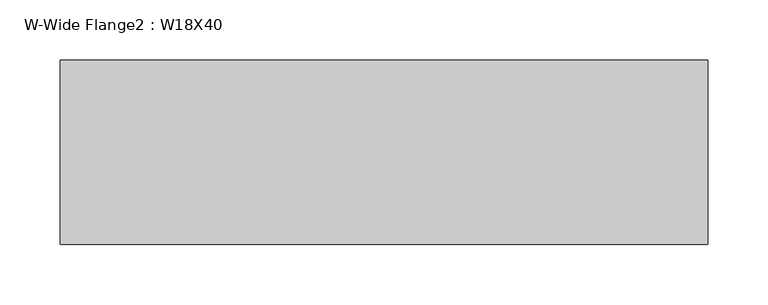
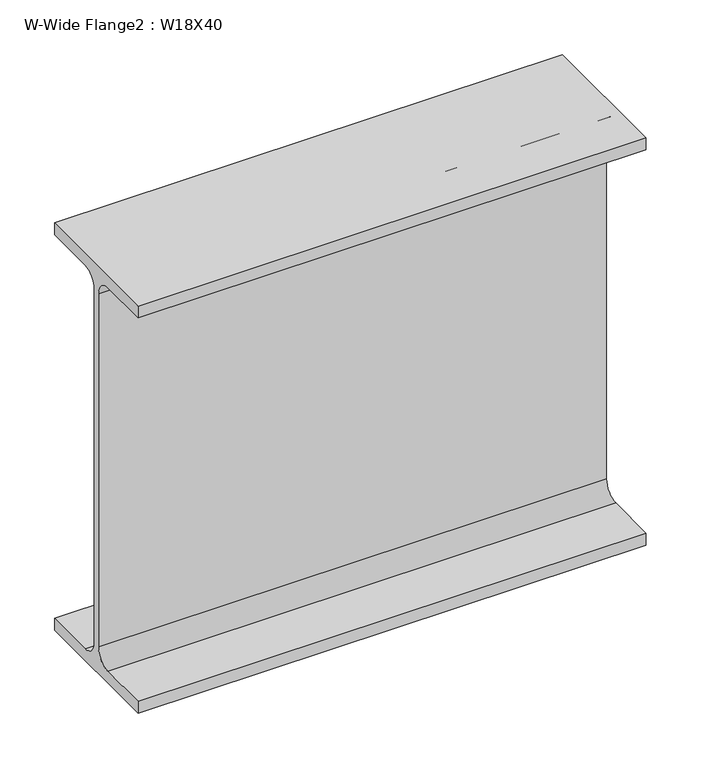
"""IFC4 building model written with IfcOpenShell, lengths in millimetres: beam geometry, W-Wide Flange2 : W18X40."""

from ifc_helpers import new_model, si_unit, point, frame, frame_2d, origin, place, context, project, spatial, polyline, circle_curve, trimmed, segment, composite_curve, outline, extrude, source, transform, mapped, element, save


def w_wide_flange2_w18x40_37f968c4(model_context):
    return source(origin(), model_context, "Body", "SweptSolid", [
        extrude(outline(composite_curve([segment(polyline([(76.454, -213.995), (76.454, -227.33), (-76.454, -227.33), (-76.454, -213.995), (-20.828, -213.995)]), True, "CONTINUOUS"), segment(trimmed(circle_curve(frame_2d((-20.828, -197.1675)), 16.8275), [point((-20.828, -213.995))], [point((-4.0005, -197.1675))], True, "CARTESIAN"), True, "CONTINUOUS"), segment(polyline([(-4.0005, -197.1675), (-4.0005, 197.1675)]), True, "CONTINUOUS"), segment(trimmed(circle_curve(frame_2d((-20.828, 197.1675)), 16.8275), [point((-4.0005, 197.1675))], [point((-20.828, 213.995))], True, "CARTESIAN"), True, "CONTINUOUS"), segment(polyline([(-20.828, 213.995), (-76.454, 213.995), (-76.454, 227.33), (76.454, 227.33), (76.454, 213.995), (20.828, 213.995)]), True, "CONTINUOUS"), segment(trimmed(circle_curve(frame_2d((20.828, 197.1675)), 16.8275), [point((20.828, 213.995))], [point((4.0005, 197.1675))], True, "CARTESIAN"), True, "CONTINUOUS"), segment(polyline([(4.0005, 197.1675), (4.0005, -197.1675)]), True, "CONTINUOUS"), segment(trimmed(circle_curve(frame_2d((20.828, -197.1675)), 16.8275), [point((4.0005, -197.1675))], [point((20.828, -213.995))], True, "CARTESIAN"), True, "CONTINUOUS"), segment(polyline([(20.828, -213.995), (76.454, -213.995)]), True, "CONTINUOUS")], self_intersect=False)), frame((-296.8625, 0.0, 0.0), z_axis=(1.0, 0.0, 0.0), x_axis=(0.0, 1.0, 0.0)), (0.0, 0.0, 1.0), 536.575),
    ])


if __name__ == "__main__":
    model = new_model("IFC4")
    model_context = context("Model", 3, world=origin())
    ifc_project = project(units=[si_unit("LENGTHUNIT", "METRE", prefix="MILLI")], contexts=[model_context])
    site = spatial("IfcSite", under=ifc_project)
    building = spatial("IfcBuilding", under=site)
    placement = place(None, origin())
    w_wide_flange2_w18x40_shape = w_wide_flange2_w18x40_37f968c4(model_context)
    element("IfcBeam", 1, ObjectType="W-Wide Flange2 : W18X40", at=placement, inside=building, context=model_context, shape_type="MappedRepresentation", body=[
        mapped(w_wide_flange2_w18x40_shape, transform((0.0, 0.0, 0.0), x_axis=(1.0, 0.0, 0.0), y_axis=(0.0, 1.0, 0.0), z_axis=(0.0, 0.0, 1.0))),
    ])
    save(model, "model.ifc")

# Revit data of these elements
# Type "W-Wide Flange2 : W18X40"
#   Assembly Code = "B10"
#   W = 40
#   Length [instance default] = 5' - 0"
#   bf = 0' - 6.02"
#   d = 1' - 5.9"
#   k = 0' - 1 3/16"
#   k2 = 0' - 0.6625"
#   tf = 0' - 0.525"
#   tw = 0' - 0.315"
#   A = 0.0819444 SF
#   Structural Material [instance default] = Steel ASTM A992
# Element 1 (IfcBeam, "W-Wide Flange2 : W18X40")
#   Materials on its faces: "Steel ASTM A992"
# Materials
#   "Steel ASTM A992": class "Metal", colour RGB 199 199 199, transparency 0, Description = "Structural steel 50ksi", Cost = 0
